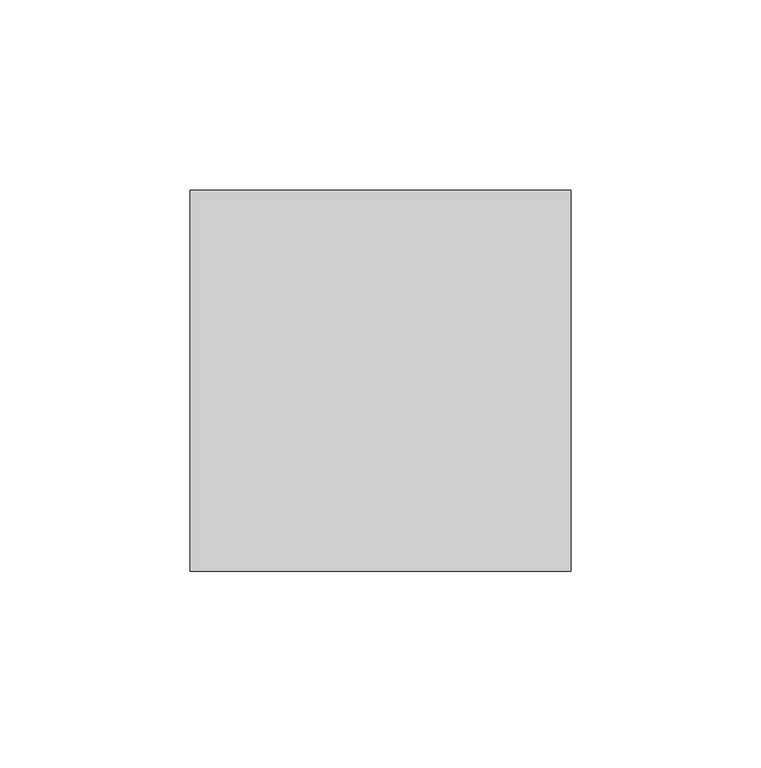
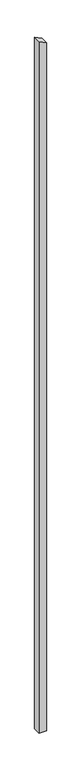
"""IFC4 building model written with IfcOpenShell, lengths in millimetres: column geometry, Holzstütze 159556 : Holzstütze 159556."""

import ifcopenshell
import ifcopenshell.guid

model = None  # the IFC model being written
_history = None  # IfcOwnerHistory: only IFC2X3 demands one
_inside = {}  # id of a spatial element -> (the spatial element, [elements in it])
_under = {}  # id of a project, library or spatial element -> (it, [spatial elements below it])
_declared = {}  # id of a project -> (the project, [libraries it declares])
_typed = {}  # id of a type object -> (the type object, [elements of that type])
_made_of = {}  # id of a material, layer set ... -> (it, [elements and type objects made of it])


def new_model(schema):
    """Start an empty IFC model of exactly this schema.

    Asked for "IFC4X3", IfcOpenShell would pick the latest addendum, in which some entities
    have other attributes; the version numbers below select the first issue.
    IFC2X3 requires an IfcOwnerHistory on every rooted entity: one is made here for all.
    """
    global model, _history
    if schema == "IFC4X3":
        model = ifcopenshell.file(schema_version=(4, 3, 0, 0))
    else:
        model = ifcopenshell.file(schema=schema)
    _inside.clear()
    _under.clear()
    _declared.clear()
    _typed.clear()
    _made_of.clear()
    _history = None
    if model.schema == "IFC2X3":
        org = make("IfcOrganization", Name="unknown")
        user = make(
            "IfcPersonAndOrganization",
            ThePerson=make("IfcPerson", FamilyName="unknown"),
            TheOrganization=org,
        )
        app = make(
            "IfcApplication",
            ApplicationDeveloper=org,
            Version="unknown",
            ApplicationFullName="unknown",
            ApplicationIdentifier="unknown",
        )
        _history = make(
            "IfcOwnerHistory",
            OwningUser=user,
            OwningApplication=app,
            ChangeAction="ADDED",
            CreationDate=0,
        )
    return model


def make(cls, **values):
    """One entity of the class cls with the attributes given. An attribute that is None is left unset."""
    return model.create_entity(
        cls, **{name: value for name, value in values.items() if value is not None}
    )


def rooted(cls, **values):
    """An entity with a GlobalId (a new one), such as an element, a storey or a relation."""
    return make(cls, GlobalId=ifcopenshell.guid.new(), OwnerHistory=_history, **values)


def si_unit(unit_type, name, prefix=None):
    """IfcSIUnit, for example si_unit("LENGTHUNIT", "METRE", prefix="MILLI")."""
    return make("IfcSIUnit", UnitType=unit_type, Prefix=prefix, Name=name)


def assignment(units):
    """IfcUnitAssignment: the units of a project."""
    return None if units is None else make("IfcUnitAssignment", Units=units)


def point(xyz):
    """IfcCartesianPoint."""
    return None if xyz is None else make("IfcCartesianPoint", Coordinates=xyz)


def direction(xyz):
    """IfcDirection."""
    return None if xyz is None else make("IfcDirection", DirectionRatios=xyz)


def frame(location, z_axis=None, x_axis=None):
    """IfcAxis2Placement3D, a coordinate frame: its origin and axes. An axis left out is left unset."""
    return make(
        "IfcAxis2Placement3D",
        Location=point(location),
        Axis=direction(z_axis),
        RefDirection=direction(x_axis),
    )


def origin():
    """The frame at (0, 0, 0) with its axes left unset."""
    return frame((0.0, 0.0, 0.0))


def place(relative_to, where):
    """IfcLocalPlacement: puts the frame where relative to a parent placement (None: the world)."""
    return make(
        "IfcLocalPlacement", PlacementRelTo=relative_to, RelativePlacement=where
    )


def context(
    kind, dimensions, precision=None, world=None, true_north=None, identifier=None
):
    """IfcGeometricRepresentationContext, for example the 3D "Model" context."""
    return make(
        "IfcGeometricRepresentationContext",
        ContextIdentifier=identifier,
        ContextType=kind,
        CoordinateSpaceDimension=dimensions,
        Precision=precision,
        WorldCoordinateSystem=world,
        TrueNorth=true_north,
    )


def project(units=None, contexts=None):
    """IfcProject with its units and contexts."""
    return rooted(
        "IfcProject",
        Name="project",
        RepresentationContexts=contexts,
        UnitsInContext=assignment(units),
    )


def spatial(cls, under=None, at=None, **own):
    """A site, building, storey or space (cls), placed at a placement, below another one or the project."""
    s = rooted(cls, ObjectPlacement=at, **own)
    if under is not None:
        _under.setdefault(under.id(), (under, []))[1].append(s)
    return s


def polyline(points):
    """IfcPolyline through the points."""
    return make("IfcPolyline", Points=[point(p) for p in points])


def outline(outer, holes=None, kind="AREA"):
    """IfcArbitraryClosedProfileDef: a profile drawn as a closed curve; with holes, ...WithVoids."""
    if holes is None:
        return make("IfcArbitraryClosedProfileDef", ProfileType=kind, OuterCurve=outer)
    return make(
        "IfcArbitraryProfileDefWithVoids",
        ProfileType=kind,
        OuterCurve=outer,
        InnerCurves=holes,
    )


def extrude(swept, where, along, depth):
    """IfcExtrudedAreaSolid: the profile swept, set in the frame where, extruded along a direction by depth."""
    return make(
        "IfcExtrudedAreaSolid",
        SweptArea=swept,
        Position=where,
        ExtrudedDirection=direction(along),
        Depth=depth,
    )


def shape(context_of_items, identifier, shape_type, items):
    """IfcShapeRepresentation: the items that make up one representation, for example the "Body"."""
    return make(
        "IfcShapeRepresentation",
        ContextOfItems=context_of_items,
        RepresentationIdentifier=identifier,
        RepresentationType=shape_type,
        Items=items,
    )


def source(mapping_origin, context_of_items, identifier, shape_type, items):
    """IfcRepresentationMap: a shape defined once, which mapped items show again and again."""
    return make(
        "IfcRepresentationMap",
        MappingOrigin=mapping_origin,
        MappedRepresentation=shape(context_of_items, identifier, shape_type, items),
    )


def transform(
    local_origin,
    x_axis=None,
    y_axis=None,
    z_axis=None,
    scale=None,
    scale2=None,
    scale3=None,
    uniform=True,
):
    """IfcCartesianTransformationOperator3D, or its non-uniform kind. x_axis, y_axis, z_axis: its Axis1, 2, 3."""
    if uniform:
        return make(
            "IfcCartesianTransformationOperator3D",
            Axis1=direction(x_axis),
            Axis2=direction(y_axis),
            LocalOrigin=point(local_origin),
            Scale=scale,
            Axis3=direction(z_axis),
        )
    return make(
        "IfcCartesianTransformationOperator3DnonUniform",
        Axis1=direction(x_axis),
        Axis2=direction(y_axis),
        LocalOrigin=point(local_origin),
        Scale=scale,
        Axis3=direction(z_axis),
        Scale2=scale2,
        Scale3=scale3,
    )


def mapped(mapping_source, mapping_target):
    """IfcMappedItem: shows the shape of a source again, moved by a transform."""
    return make(
        "IfcMappedItem", MappingSource=mapping_source, MappingTarget=mapping_target
    )


def made_of(thing, what):
    """Note that an element or type object is made of a material, layer set ...; save() writes the relation."""
    if what is not None:
        _made_of.setdefault(what.id(), (what, []))[1].append(thing)
    return thing


def element(
    cls,
    number,
    at=None,
    inside=None,
    cuts=None,
    type_object=None,
    material=None,
    context=None,
    identifier="Body",
    shape_type=None,
    held_by="IfcProductDefinitionShape",
    body=None,
    shapes=None,
    **own,
):
    """One element of the class cls, such as IfcWall. Its Tag is "e" and its number.

    at: its placement. inside: the storey or other place that contains it. cuts: it is an
    opening in that element (IfcRelVoidsElement). A single representation is given by context,
    identifier, shape_type and body (its items); several are given by shapes. held_by: the class
    of the entity that holds the representations. save() writes the other relations.
    """
    e = rooted(cls, Tag="e%d" % number, ObjectPlacement=at, **own)
    if body is not None:
        shapes = [shape(context, identifier, shape_type, body)]
    if shapes is not None:
        e.Representation = make(held_by, Representations=shapes)
    if inside is not None:
        _inside.setdefault(inside.id(), (inside, []))[1].append(e)
    if cuts is not None:
        rooted(
            "IfcRelVoidsElement", RelatingBuildingElement=cuts, RelatedOpeningElement=e
        )
    if type_object is not None:
        _typed.setdefault(type_object.id(), (type_object, []))[1].append(e)
    return made_of(e, material)


def aggregate(whole, parts):
    """IfcRelAggregates: a whole, such as a stair, and the parts it consists of."""
    return rooted("IfcRelAggregates", RelatingObject=whole, RelatedObjects=parts)


def save(model, path):
    """Write the relations noted so far, then the file.

    IfcRelAggregates (storeys below a building ...), IfcRelContainedInSpatialStructure (elements
    in a storey), IfcRelDefinesByType, IfcRelAssociatesMaterial and IfcRelDeclares: one each for
    every whole, place, type object, material and project.
    """
    for whole, parts in _under.values():
        aggregate(whole, parts)
    for where, things in _inside.values():
        rooted(
            "IfcRelContainedInSpatialStructure",
            RelatedElements=things,
            RelatingStructure=where,
        )
    for kind, things in _typed.values():
        rooted("IfcRelDefinesByType", RelatedObjects=things, RelatingType=kind)
    for what, things in _made_of.values():
        rooted("IfcRelAssociatesMaterial", RelatedObjects=things, RelatingMaterial=what)
    for by, libraries in _declared.values():
        rooted("IfcRelDeclares", RelatingContext=by, RelatedDefinitions=libraries)
    model.write(path)


def column_44b88cc2(model_context):
    return source(origin(), model_context, "Body", "SweptSolid", [
        extrude(outline(polyline([(-500.0, 168257.7593015), (-500.0, 168357.7593015), (9372.2929958, 168357.7593015), (9423.2455407, 168257.7593015), (-500.0, 168257.7593015)])), frame((0.0, 26981.9343946, 0.0), z_axis=(0.0, 1.0, 0.0), x_axis=(0.0, 0.0, 1.0)), (0.0, 0.0, 1.0), 100.0),
    ])


if __name__ == "__main__":
    model = new_model("IFC4")
    model_context = context("Model", 3, world=origin())
    ifc_project = project(units=[si_unit("LENGTHUNIT", "METRE", prefix="MILLI")], contexts=[model_context])
    site = spatial("IfcSite", under=ifc_project)
    building = spatial("IfcBuilding", under=site)
    placement = place(None, origin())
    column_shape = column_44b88cc2(model_context)
    element("IfcColumn", 1, ObjectType="Holzstütze 159556 : Holzstütze 159556", at=placement, inside=building, context=model_context, shape_type="MappedRepresentation", body=[
        mapped(column_shape, transform((0.0, 0.0, 0.0), x_axis=(1.0, 0.0, 0.0), y_axis=(0.0, 1.0, 0.0), z_axis=(0.0, 0.0, 1.0))),
    ])
    save(model, "model.ifc")

# Revit data of these elements
# Type "Holzstütze 159556 : Holzstütze 159556"
#   Abrechnungsart = "m"
#   Allright_Bauteil_ID = "0152St 0000143461"
#   Bezeichnung = "Holzstütze"
#   Codetext = "ST-HOLZ\\"
#   Gewerk = "Zimmer- und Holzbauarbeiten"
#   Material = "Holz"
#   Objektname = "Stütze"
#   NameOverride = "Holzstütze"
#   Reference = "Holzstütze"
#   Status = "NEW"
#   ThermalTransmittance = 0.0000 BTU/(h·ft²·°F)
#   Roll = 0.00°
#   Slope = 0.00°
#   2D Interaktion = yes
#   IsExternal = yes
#   LoadBearing = yes
# Element 1 (IfcColumn, "Holzstütze 159556 : Holzstütze 159556")
#   Materials on its faces: "holzschalung"
# Materials
#   "holzschalung": class "Unassigned", colour RGB 128 128 128, transparency 0
